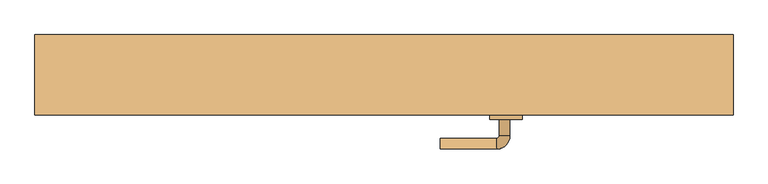
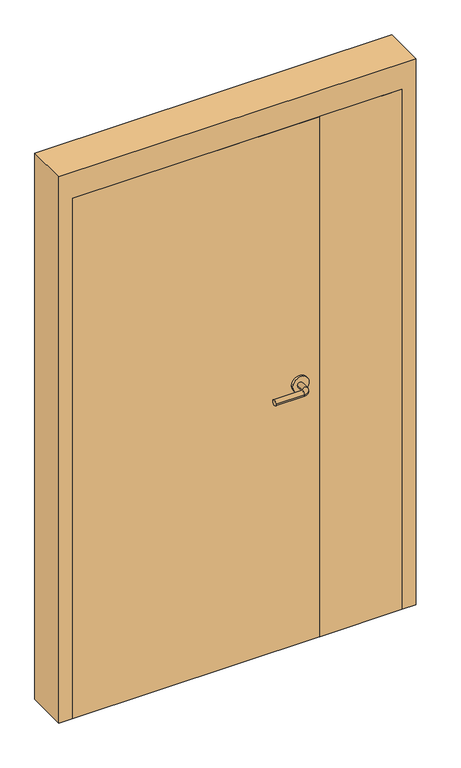
"""IFC4 building model written with IfcOpenShell, lengths in millimetres: door geometry, Дверь-Маятниковая-С полотнами разной ширины-Щитовая : 1300 x 2100 мм."""

from ifc_helpers import new_model, si_unit, point, frame, frame_2d, origin, origin_with_axes, place, context, project, spatial, polyline, circle_curve, ellipse_curve, trimmed, segment, composite_curve, outline, extrude, faceted_brep, source, transform, mapped, element, save
from ifc_brep_helpers import plane_surface, cylinder_surface, revolved_surface, advanced_brep


def door_bf617f1b(model_context):
    return source(origin(), model_context, "Body", "SolidModel", [
        advanced_brep(
        [(234.59375, -15.85, 1000.0), (214.59375, -15.85, 1000.0), (214.59375, 14.15, 1000.0), (234.59375, 14.15, 1000.0), (209.59375, 19.15, 1000.0), (209.59375, 39.15, 1000.0), (104.59375, 39.15, 1000.0), (104.59375, 19.15, 1000.0)],
        [
            (0, 1, circle_curve(frame((224.59375, -15.85, 1000.0), z_axis=(0.0, -1.0, 0.0), x_axis=(-1.0, 0.0, 0.0)), 10.0)),
            (1, 0, circle_curve(frame((224.59375, -15.85, 1000.0), z_axis=(0.0, -1.0, 0.0), x_axis=(-1.0, 0.0, 0.0)), 10.0)),
            (1, 2),
            (2, 3, circle_curve(frame((224.59375, 14.15, 1000.0), z_axis=(0.0, -1.0, 0.0), x_axis=(-1.0, 0.0, 0.0)), 10.0)),
            (3, 0),
            (3, 2, circle_curve(frame((224.59375, 14.15, 1000.0), z_axis=(0.0, -1.0, 0.0), x_axis=(-1.0, 0.0, 0.0)), 10.0)),
            (4, 5, circle_curve(frame((209.59375, 29.15, 1000.0), z_axis=(1.0, 0.0, 0.0), x_axis=(0.0, -1.0, 0.0)), 10.0)),
            (5, 3, circle_curve(frame((209.59375, 14.15, 1000.0), z_axis=(0.0, 0.0, -1.0), x_axis=(1.0, 0.0, 0.0)), 25.0)),
            (2, 4, circle_curve(frame((209.59375, 14.15, 1000.0), z_axis=(0.0, 0.0, 1.0), x_axis=(1.0, 0.0, 0.0)), 5.0)),
            (5, 4, circle_curve(frame((209.59375, 29.15, 1000.0), z_axis=(1.0, 0.0, 0.0), x_axis=(0.0, -1.0, 0.0)), 10.0)),
            (6, 7, circle_curve(frame((104.59375, 29.15, 1000.0), z_axis=(-1.0, 0.0, 0.0), x_axis=(0.0, -1.0, 0.0)), 10.0)),
            (7, 6, circle_curve(frame((104.59375, 29.15, 1000.0), z_axis=(-1.0, 0.0, 0.0), x_axis=(0.0, -1.0, 0.0)), 10.0)),
            (4, 7),
            (6, 5),
        ],
        [
            plane_surface(frame((224.59375, -15.85, 1000.0), z_axis=(0.0, -1.0, 0.0), x_axis=(0.0, 0.0, 1.0))),
            cylinder_surface(frame((224.59375, -15.85, 1000.0), z_axis=(0.0, -1.0, 0.0), x_axis=(-1.0, 0.0, 0.0)), 10.0),
            revolved_surface(trimmed(ellipse_curve(frame((224.59375, 14.15, 1000.0), z_axis=(0.0, 1.0, 0.0), x_axis=(-1.0, 0.0, 0.0)), 10.0, 10.0), [point((234.59375, 14.15, 1000.0))], [point((214.59375, 14.15, 1000.0))], True, "CARTESIAN"), (209.59375, 14.15, 1000.0), (0.0, 0.0, -1.0)),
            revolved_surface(trimmed(ellipse_curve(frame((224.59375, 14.15, 1000.0), z_axis=(0.0, 1.0, 0.0), x_axis=(-1.0, 0.0, 0.0)), 10.0, 10.0), [point((214.59375, 14.15, 1000.0))], [point((234.59375, 14.15, 1000.0))], True, "CARTESIAN"), (209.59375, 14.15, 1000.0), (0.0, 0.0, -1.0)),
            plane_surface(frame((104.59375, 29.15, 1000.0), z_axis=(-1.0, 0.0, 0.0), x_axis=(0.0, 0.0, 1.0))),
            cylinder_surface(frame((209.59375, 29.15, 1000.0), z_axis=(1.0, 0.0, 0.0), x_axis=(0.0, -1.0, 0.0)), 10.0),
        ],
        [
            (0, [[1, 2]]),
            (1, [[3, 4, 5, -2]]),
            (1, [[-5, 6, -3, -1]]),
            (2, [[7, 8, -4, 9]]),
            (3, [[10, -9, -6, -8]]),
            (4, [[11, 12]]),
            (5, [[13, -11, 14, -7]]),
            (5, [[-14, -12, -13, -10]]),
        ],
    ),
        extrude(outline(composite_curve([segment(trimmed(circle_curve(frame_2d((1000.0, 227.09375)), 30.0), [point((1000.0, 257.09375))], [point((1000.0, 197.09375))], False, "CARTESIAN"), True, "CONTINUOUS"), segment(trimmed(circle_curve(frame_2d((1000.0, 227.09375)), 30.0), [point((1000.0, 197.09375))], [point((1000.0, 257.09375))], False, "CARTESIAN"), True, "CONTINUOUS")], self_intersect=False)), frame((0.0, -23.85, 0.0), z_axis=(0.0, 1.0, 0.0), x_axis=(0.0, 0.0, 1.0)), (0.0, 0.0, 1.0), 8.0),
        advanced_brep(
        [(234.59375, -76.85, 1000.0), (214.59375, -76.85, 1000.0), (234.59375, -106.85, 1000.0), (214.59375, -106.85, 1000.0), (209.59375, -111.85, 1000.0), (209.59375, -131.85, 1000.0), (104.59375, -131.85, 1000.0), (104.59375, -111.85, 1000.0)],
        [
            (0, 1, circle_curve(frame((224.59375, -76.85, 1000.0), z_axis=(0.0, 1.0, 0.0), x_axis=(-1.0, 0.0, 0.0)), 10.0)),
            (1, 0, circle_curve(frame((224.59375, -76.85, 1000.0), z_axis=(0.0, 1.0, 0.0), x_axis=(-1.0, 0.0, 0.0)), 10.0)),
            (0, 2),
            (2, 3, circle_curve(frame((224.59375, -106.85, 1000.0), z_axis=(0.0, 1.0, 0.0), x_axis=(-1.0, 0.0, 0.0)), 10.0)),
            (3, 1),
            (3, 2, circle_curve(frame((224.59375, -106.85, 1000.0), z_axis=(0.0, 1.0, 0.0), x_axis=(-1.0, 0.0, 0.0)), 10.0)),
            (4, 3, circle_curve(frame((209.59375, -106.85, 1000.0), z_axis=(0.0, 0.0, 1.0), x_axis=(1.0, 0.0, 0.0)), 5.0)),
            (2, 5, circle_curve(frame((209.59375, -106.85, 1000.0), z_axis=(0.0, 0.0, -1.0), x_axis=(1.0, 0.0, 0.0)), 25.0)),
            (5, 4, circle_curve(frame((209.59375, -121.85, 1000.0), z_axis=(1.0, 0.0, 0.0), x_axis=(0.0, 1.0, 0.0)), 10.0)),
            (4, 5, circle_curve(frame((209.59375, -121.85, 1000.0), z_axis=(1.0, 0.0, 0.0), x_axis=(0.0, 1.0, 0.0)), 10.0)),
            (6, 7, circle_curve(frame((104.59375, -121.85, 1000.0), z_axis=(-1.0, 0.0, 0.0), x_axis=(0.0, 1.0, 0.0)), 10.0)),
            (7, 6, circle_curve(frame((104.59375, -121.85, 1000.0), z_axis=(-1.0, 0.0, 0.0), x_axis=(0.0, 1.0, 0.0)), 10.0)),
            (5, 6),
            (7, 4),
        ],
        [
            plane_surface(frame((224.59375, -76.85, 1000.0), z_axis=(0.0, 1.0, 0.0), x_axis=(0.0, 0.0, 1.0))),
            cylinder_surface(frame((224.59375, -76.85, 1000.0), z_axis=(0.0, 1.0, 0.0), x_axis=(-1.0, 0.0, 0.0)), 10.0),
            revolved_surface(trimmed(ellipse_curve(frame((224.59375, -106.85, 1000.0), z_axis=(0.0, 1.0, 0.0), x_axis=(-1.0, 0.0, 0.0)), 10.0, 10.0), [point((234.59375, -106.85, 1000.0))], [point((214.59375, -106.85, 1000.0))], True, "CARTESIAN"), (209.59375, -106.85, 1000.0), (0.0, 0.0, -1.0)),
            revolved_surface(trimmed(ellipse_curve(frame((224.59375, -106.85, 1000.0), z_axis=(0.0, 1.0, 0.0), x_axis=(-1.0, 0.0, 0.0)), 10.0, 10.0), [point((214.59375, -106.85, 1000.0))], [point((234.59375, -106.85, 1000.0))], True, "CARTESIAN"), (209.59375, -106.85, 1000.0), (0.0, 0.0, -1.0)),
            plane_surface(frame((104.59375, -121.85, 1000.0), z_axis=(-1.0, 0.0, 0.0), x_axis=(0.0, 0.0, 1.0))),
            cylinder_surface(frame((209.59375, -121.85, 1000.0), z_axis=(1.0, 0.0, 0.0), x_axis=(0.0, 1.0, 0.0)), 10.0),
        ],
        [
            (0, [[1, 2]]),
            (1, [[-1, 3, 4, 5]]),
            (1, [[-2, -5, 6, -3]]),
            (2, [[7, -4, 8, 9]]),
            (3, [[-8, -6, -7, 10]]),
            (4, [[11, 12]]),
            (5, [[-9, 13, -12, 14]]),
            (5, [[-10, -14, -11, -13]]),
        ],
    ),
        extrude(outline(composite_curve([segment(trimmed(circle_curve(frame_2d((1000.0, 227.09375)), 30.0), [point((1000.0, 257.09375))], [point((1000.0, 197.09375))], False, "CARTESIAN"), True, "CONTINUOUS"), segment(trimmed(circle_curve(frame_2d((1000.0, 227.09375)), 30.0), [point((1000.0, 197.09375))], [point((1000.0, 257.09375))], False, "CARTESIAN"), True, "CONTINUOUS")], self_intersect=False)), frame((0.0, -76.85, 0.0), z_axis=(0.0, 1.0, 0.0), x_axis=(0.0, 0.0, 1.0)), (0.0, 0.0, 1.0), 8.0),
        extrude(outline(polyline([(600.0, -23.85), (600.0, -68.85), (301.6, -68.85), (301.6, -23.85), (600.0, -23.85)])), origin_with_axes(), (0.0, 0.0, 1.0), 2000.0),
        faceted_brep([(600.0, -19.0875, 0.0), (584.125, -19.0875, 0.0), (584.125, 31.9375, 0.0), (600.0, 31.9375, 0.0), (600.0, 81.15, 0.0), (650.0, 81.15, 0.0), (650.0, -68.85, 0.0), (600.0, -68.85, 0.0), (600.0, -68.85, 2000.0), (600.0, -19.0875, 2000.0), (650.0, -68.85, 2100.0), (-650.0, -68.85, 2100.0), (-650.0, -68.85, 0.0), (-600.0, -68.85, 0.0), (-600.0, -68.85, 2000.0), (650.0, 81.15, 2100.0), (600.0, 81.15, 2000.0), (-600.0, 81.15, 2000.0), (-600.0, 81.15, 0.0), (-650.0, 81.15, 0.0), (-650.0, 81.15, 2100.0), (600.0, 31.9375, 2000.0), (584.125, 31.9375, 1984.125), (-584.125, 31.9375, 1984.125), (-584.125, 31.9375, 0.0), (-600.0, 31.9375, 0.0), (-600.0, 31.9375, 2000.0), (584.125, -19.0875, 1984.125), (-600.0, -19.0875, 2000.0), (-600.0, -19.0875, 0.0), (-584.125, -19.0875, 0.0), (-584.125, -19.0875, 1984.125)], [[[0, 1, 2, 3, 4, 5, 6, 7]], [[7, 8, 9, 0]], [[6, 10, 11, 12, 13, 14, 8, 7]], [[5, 15, 10, 6]], [[4, 16, 17, 18, 19, 20, 15, 5]], [[3, 21, 16, 4]], [[2, 22, 23, 24, 25, 26, 21, 3]], [[1, 27, 22, 2]], [[0, 9, 28, 29, 30, 31, 27, 1]], [[8, 14, 28, 9]], [[16, 21, 26, 17]], [[22, 27, 31, 23]], [[12, 19, 18, 25, 24, 30, 29, 13]], [[13, 29, 28, 14]], [[11, 20, 19, 12]], [[17, 26, 25, 18]], [[23, 31, 30, 24]], [[15, 20, 11, 10]]]),
        extrude(outline(polyline([(298.4, -23.85), (298.4, -68.85), (-600.0, -68.85), (-600.0, -23.85), (298.4, -23.85)])), origin_with_axes(), (0.0, 0.0, 1.0), 2000.0),
    ])


if __name__ == "__main__":
    model = new_model("IFC4")
    model_context = context("Model", 3, world=origin())
    ifc_project = project(units=[si_unit("LENGTHUNIT", "METRE", prefix="MILLI")], contexts=[model_context])
    site = spatial("IfcSite", under=ifc_project)
    building = spatial("IfcBuilding", under=site)
    placement = place(None, origin())
    door_shape = door_bf617f1b(model_context)
    element("IfcDoor", 1, ObjectType="Дверь-Маятниковая-С полотнами разной ширины-Щитовая : 1300 x 2100 мм", at=placement, inside=building, context=model_context, shape_type="MappedRepresentation", body=[
        mapped(door_shape, transform((0.0, 0.0, 0.0), x_axis=(1.0, 0.0, 0.0), y_axis=(0.0, 1.0, 0.0), z_axis=(0.0, 0.0, 1.0))),
    ])
    save(model, "model.ifc")

# Revit data of these elements
# Type "Дверь-Маятниковая-С полотнами разной ширины-Щитовая : 1300 x 2100 мм"
#   Type Mark = "144"
#   Assembly Code = "C1020300"
#   Analytic Construction = "Деревянный"
#   Ширина большой панели = 900 mm
#   W = 300 mm
#   Thickness = 45 mm
#   Thermal Resistance (R) = 0.455703 (m²·K)/W
#   Угол поворота [instance default] = 90°
#   Высота планки = 1000 mm
#   Rough Width [instance default] = 1300 mm
#   Rough Height [instance default] = 2100 mm
#   Высота проема в кирпичном каркасе [instance default] = 100 mm
#   Ширина проема в кирпичном каркасе [instance default] = 100 mm
#   Расчет вставки [instance default] = 105 mm
#   Кирпичная вставка [instance default] = 25 mm
#   Height = 2000 mm
#   Width = 1200 mm
#   Heat Transfer Coefficient (U) = 2.19465 W/(m²·K)
#   Глубина кирпичного каркаса = 150 mm
#   Кирпичный каркас [instance default] = yes
#   Каркас стены сухой кладки [instance default] = no
#   Материал панели = Древесина - Береза
#   Материал каркаса = Металл - Окрашенный - Серый 2
#   Материал дверной ручки = Алюминий
#   Visual Light Transmittance = 0
#   Solar Heat Gain Coefficient = 0
#   Wall Closure = (empty or 0)
#   Function = (empty or 0)
# Element 1 (IfcDoor, "Дверь-Маятниковая-С полотнами разной ширины-Щитовая : 1300 x 2100 мм")
#   Расчет вставки = 80 mm
#   Кирпичная вставка = 0 mm
#   Materials on its faces: "Алюминий", "Металл - Окрашенный - Серый 2", "Древесина - Береза"
# Materials
#   "Древесина - Береза": class "Древесина", colour RGB 166 116 52, transparency 0, Cost = 0
#   "Металл - Окрашенный - Серый 2": class "Краска", colour RGB 104 104 104, transparency 0, Cost = 0
#   "Алюминий": class "Металл", colour RGB 247 247 247, transparency 0
